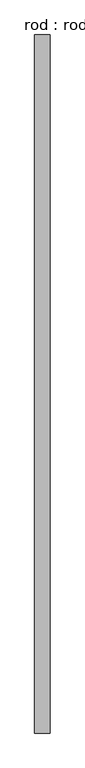
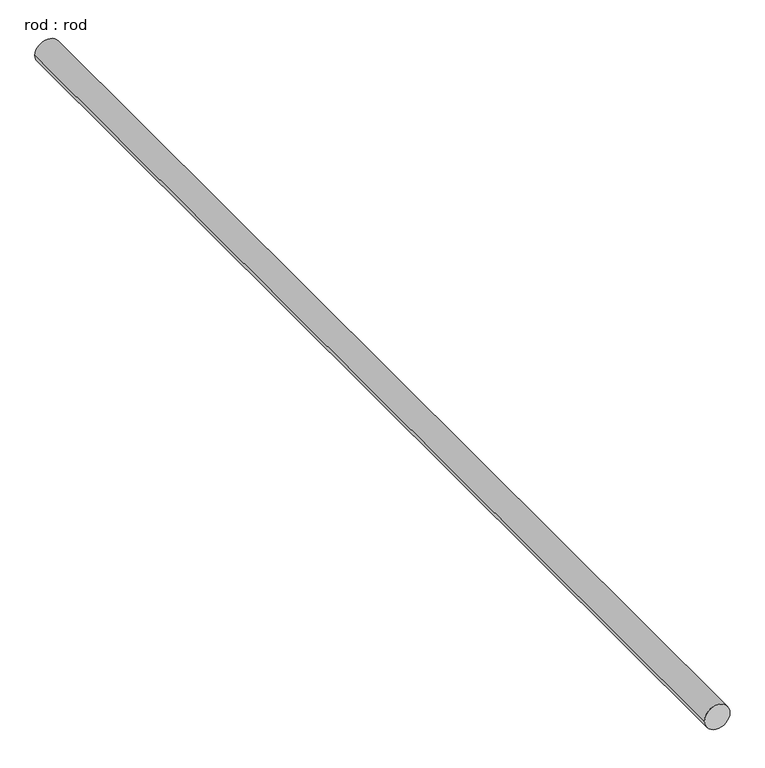
"""IFC4 building model written with IfcOpenShell, lengths in millimetres: proxy geometry, rod : rod."""

import ifcopenshell
import ifcopenshell.guid

model = None  # the IFC model being written
_history = None  # IfcOwnerHistory: only IFC2X3 demands one
_inside = {}  # id of a spatial element -> (the spatial element, [elements in it])
_under = {}  # id of a project, library or spatial element -> (it, [spatial elements below it])
_declared = {}  # id of a project -> (the project, [libraries it declares])
_typed = {}  # id of a type object -> (the type object, [elements of that type])
_made_of = {}  # id of a material, layer set ... -> (it, [elements and type objects made of it])


def new_model(schema):
    """Start an empty IFC model of exactly this schema.

    Asked for "IFC4X3", IfcOpenShell would pick the latest addendum, in which some entities
    have other attributes; the version numbers below select the first issue.
    IFC2X3 requires an IfcOwnerHistory on every rooted entity: one is made here for all.
    """
    global model, _history
    if schema == "IFC4X3":
        model = ifcopenshell.file(schema_version=(4, 3, 0, 0))
    else:
        model = ifcopenshell.file(schema=schema)
    _inside.clear()
    _under.clear()
    _declared.clear()
    _typed.clear()
    _made_of.clear()
    _history = None
    if model.schema == "IFC2X3":
        org = make("IfcOrganization", Name="unknown")
        user = make(
            "IfcPersonAndOrganization",
            ThePerson=make("IfcPerson", FamilyName="unknown"),
            TheOrganization=org,
        )
        app = make(
            "IfcApplication",
            ApplicationDeveloper=org,
            Version="unknown",
            ApplicationFullName="unknown",
            ApplicationIdentifier="unknown",
        )
        _history = make(
            "IfcOwnerHistory",
            OwningUser=user,
            OwningApplication=app,
            ChangeAction="ADDED",
            CreationDate=0,
        )
    return model


def make(cls, **values):
    """One entity of the class cls with the attributes given. An attribute that is None is left unset."""
    return model.create_entity(
        cls, **{name: value for name, value in values.items() if value is not None}
    )


def rooted(cls, **values):
    """An entity with a GlobalId (a new one), such as an element, a storey or a relation."""
    return make(cls, GlobalId=ifcopenshell.guid.new(), OwnerHistory=_history, **values)


def si_unit(unit_type, name, prefix=None):
    """IfcSIUnit, for example si_unit("LENGTHUNIT", "METRE", prefix="MILLI")."""
    return make("IfcSIUnit", UnitType=unit_type, Prefix=prefix, Name=name)


def assignment(units):
    """IfcUnitAssignment: the units of a project."""
    return None if units is None else make("IfcUnitAssignment", Units=units)


def point(xyz):
    """IfcCartesianPoint."""
    return None if xyz is None else make("IfcCartesianPoint", Coordinates=xyz)


def direction(xyz):
    """IfcDirection."""
    return None if xyz is None else make("IfcDirection", DirectionRatios=xyz)


def frame(location, z_axis=None, x_axis=None):
    """IfcAxis2Placement3D, a coordinate frame: its origin and axes. An axis left out is left unset."""
    return make(
        "IfcAxis2Placement3D",
        Location=point(location),
        Axis=direction(z_axis),
        RefDirection=direction(x_axis),
    )


def frame_2d(location, x_axis=None):
    """IfcAxis2Placement2D, a coordinate frame in the plane: its origin and x axis."""
    return make(
        "IfcAxis2Placement2D", Location=point(location), RefDirection=direction(x_axis)
    )


def origin():
    """The frame at (0, 0, 0) with its axes left unset."""
    return frame((0.0, 0.0, 0.0))


def place(relative_to, where):
    """IfcLocalPlacement: puts the frame where relative to a parent placement (None: the world)."""
    return make(
        "IfcLocalPlacement", PlacementRelTo=relative_to, RelativePlacement=where
    )


def context(
    kind, dimensions, precision=None, world=None, true_north=None, identifier=None
):
    """IfcGeometricRepresentationContext, for example the 3D "Model" context."""
    return make(
        "IfcGeometricRepresentationContext",
        ContextIdentifier=identifier,
        ContextType=kind,
        CoordinateSpaceDimension=dimensions,
        Precision=precision,
        WorldCoordinateSystem=world,
        TrueNorth=true_north,
    )


def project(units=None, contexts=None):
    """IfcProject with its units and contexts."""
    return rooted(
        "IfcProject",
        Name="project",
        RepresentationContexts=contexts,
        UnitsInContext=assignment(units),
    )


def spatial(cls, under=None, at=None, **own):
    """A site, building, storey or space (cls), placed at a placement, below another one or the project."""
    s = rooted(cls, ObjectPlacement=at, **own)
    if under is not None:
        _under.setdefault(under.id(), (under, []))[1].append(s)
    return s


def circle_curve(where, radius):
    """IfcCircle in the frame where."""
    return make("IfcCircle", Position=where, Radius=radius)


def trimmed(basis, trim1, trim2, sense, master):
    """IfcTrimmedCurve: the piece of a basis curve between two trims."""
    return make(
        "IfcTrimmedCurve",
        BasisCurve=basis,
        Trim1=trim1,
        Trim2=trim2,
        SenseAgreement=sense,
        MasterRepresentation=master,
    )


def segment(curve, same_sense, transition):
    """IfcCompositeCurveSegment."""
    return make(
        "IfcCompositeCurveSegment",
        Transition=transition,
        SameSense=same_sense,
        ParentCurve=curve,
    )


def composite_curve(segments, self_intersect=None):
    """IfcCompositeCurve: segments joined end to end."""
    return make("IfcCompositeCurve", Segments=segments, SelfIntersect=self_intersect)


def outline(outer, holes=None, kind="AREA"):
    """IfcArbitraryClosedProfileDef: a profile drawn as a closed curve; with holes, ...WithVoids."""
    if holes is None:
        return make("IfcArbitraryClosedProfileDef", ProfileType=kind, OuterCurve=outer)
    return make(
        "IfcArbitraryProfileDefWithVoids",
        ProfileType=kind,
        OuterCurve=outer,
        InnerCurves=holes,
    )


def extrude(swept, where, along, depth):
    """IfcExtrudedAreaSolid: the profile swept, set in the frame where, extruded along a direction by depth."""
    return make(
        "IfcExtrudedAreaSolid",
        SweptArea=swept,
        Position=where,
        ExtrudedDirection=direction(along),
        Depth=depth,
    )


def shape(context_of_items, identifier, shape_type, items):
    """IfcShapeRepresentation: the items that make up one representation, for example the "Body"."""
    return make(
        "IfcShapeRepresentation",
        ContextOfItems=context_of_items,
        RepresentationIdentifier=identifier,
        RepresentationType=shape_type,
        Items=items,
    )


def source(mapping_origin, context_of_items, identifier, shape_type, items):
    """IfcRepresentationMap: a shape defined once, which mapped items show again and again."""
    return make(
        "IfcRepresentationMap",
        MappingOrigin=mapping_origin,
        MappedRepresentation=shape(context_of_items, identifier, shape_type, items),
    )


def transform(
    local_origin,
    x_axis=None,
    y_axis=None,
    z_axis=None,
    scale=None,
    scale2=None,
    scale3=None,
    uniform=True,
):
    """IfcCartesianTransformationOperator3D, or its non-uniform kind. x_axis, y_axis, z_axis: its Axis1, 2, 3."""
    if uniform:
        return make(
            "IfcCartesianTransformationOperator3D",
            Axis1=direction(x_axis),
            Axis2=direction(y_axis),
            LocalOrigin=point(local_origin),
            Scale=scale,
            Axis3=direction(z_axis),
        )
    return make(
        "IfcCartesianTransformationOperator3DnonUniform",
        Axis1=direction(x_axis),
        Axis2=direction(y_axis),
        LocalOrigin=point(local_origin),
        Scale=scale,
        Axis3=direction(z_axis),
        Scale2=scale2,
        Scale3=scale3,
    )


def mapped(mapping_source, mapping_target):
    """IfcMappedItem: shows the shape of a source again, moved by a transform."""
    return make(
        "IfcMappedItem", MappingSource=mapping_source, MappingTarget=mapping_target
    )


def made_of(thing, what):
    """Note that an element or type object is made of a material, layer set ...; save() writes the relation."""
    if what is not None:
        _made_of.setdefault(what.id(), (what, []))[1].append(thing)
    return thing


def element(
    cls,
    number,
    at=None,
    inside=None,
    cuts=None,
    type_object=None,
    material=None,
    context=None,
    identifier="Body",
    shape_type=None,
    held_by="IfcProductDefinitionShape",
    body=None,
    shapes=None,
    **own,
):
    """One element of the class cls, such as IfcWall. Its Tag is "e" and its number.

    at: its placement. inside: the storey or other place that contains it. cuts: it is an
    opening in that element (IfcRelVoidsElement). A single representation is given by context,
    identifier, shape_type and body (its items); several are given by shapes. held_by: the class
    of the entity that holds the representations. save() writes the other relations.
    """
    e = rooted(cls, Tag="e%d" % number, ObjectPlacement=at, **own)
    if body is not None:
        shapes = [shape(context, identifier, shape_type, body)]
    if shapes is not None:
        e.Representation = make(held_by, Representations=shapes)
    if inside is not None:
        _inside.setdefault(inside.id(), (inside, []))[1].append(e)
    if cuts is not None:
        rooted(
            "IfcRelVoidsElement", RelatingBuildingElement=cuts, RelatedOpeningElement=e
        )
    if type_object is not None:
        _typed.setdefault(type_object.id(), (type_object, []))[1].append(e)
    return made_of(e, material)


def aggregate(whole, parts):
    """IfcRelAggregates: a whole, such as a stair, and the parts it consists of."""
    return rooted("IfcRelAggregates", RelatingObject=whole, RelatedObjects=parts)


def save(model, path):
    """Write the relations noted so far, then the file.

    IfcRelAggregates (storeys below a building ...), IfcRelContainedInSpatialStructure (elements
    in a storey), IfcRelDefinesByType, IfcRelAssociatesMaterial and IfcRelDeclares: one each for
    every whole, place, type object, material and project.
    """
    for whole, parts in _under.values():
        aggregate(whole, parts)
    for where, things in _inside.values():
        rooted(
            "IfcRelContainedInSpatialStructure",
            RelatedElements=things,
            RelatingStructure=where,
        )
    for kind, things in _typed.values():
        rooted("IfcRelDefinesByType", RelatedObjects=things, RelatingType=kind)
    for what, things in _made_of.values():
        rooted("IfcRelAssociatesMaterial", RelatedObjects=things, RelatingMaterial=what)
    for by, libraries in _declared.values():
        rooted("IfcRelDeclares", RelatingContext=by, RelatedDefinitions=libraries)
    model.write(path)


def rod_rod_a6dc6763(model_context):
    return source(origin(), model_context, "Body", "SweptSolid", [
        extrude(outline(composite_curve([segment(trimmed(circle_curve(frame_2d((0.0108462, 0.0)), 200.0), [point((0.0108462, 200.0))], [point((0.0108462, -200.0))], False, "CARTESIAN"), True, "CONTINUOUS"), segment(trimmed(circle_curve(frame_2d((0.0108462, 0.0)), 200.0), [point((0.0108462, -200.0))], [point((0.0108462, 200.0))], False, "CARTESIAN"), True, "CONTINUOUS")], self_intersect=False)), frame((0.0, -5016.8573385, 0.0), z_axis=(0.0, 1.0, 0.0), x_axis=(0.0, 0.0, 1.0)), (0.0, 0.0, 1.0), 18219.1719076),
    ])


if __name__ == "__main__":
    model = new_model("IFC4")
    model_context = context("Model", 3, world=origin())
    ifc_project = project(units=[si_unit("LENGTHUNIT", "METRE", prefix="MILLI")], contexts=[model_context])
    site = spatial("IfcSite", under=ifc_project)
    building = spatial("IfcBuilding", under=site)
    placement = place(None, origin())
    rod_rod_shape = rod_rod_a6dc6763(model_context)
    element("IfcBuildingElementProxy", 1, Name="rod : rod", ObjectType="rod : rod", at=placement, inside=building, context=model_context, shape_type="MappedRepresentation", body=[
        mapped(rod_rod_shape, transform((0.0, 0.0, 0.0), x_axis=(1.0, 0.0, 0.0), y_axis=(0.0, 1.0, 0.0), z_axis=(0.0, 0.0, 1.0))),
    ])
    save(model, "model.ifc")

# Revit data of these elements
# Type "rod : rod"
#   Default Elevation = 0
